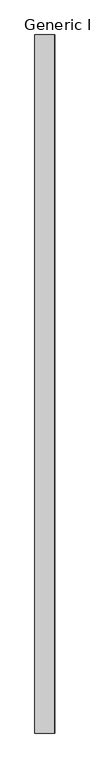
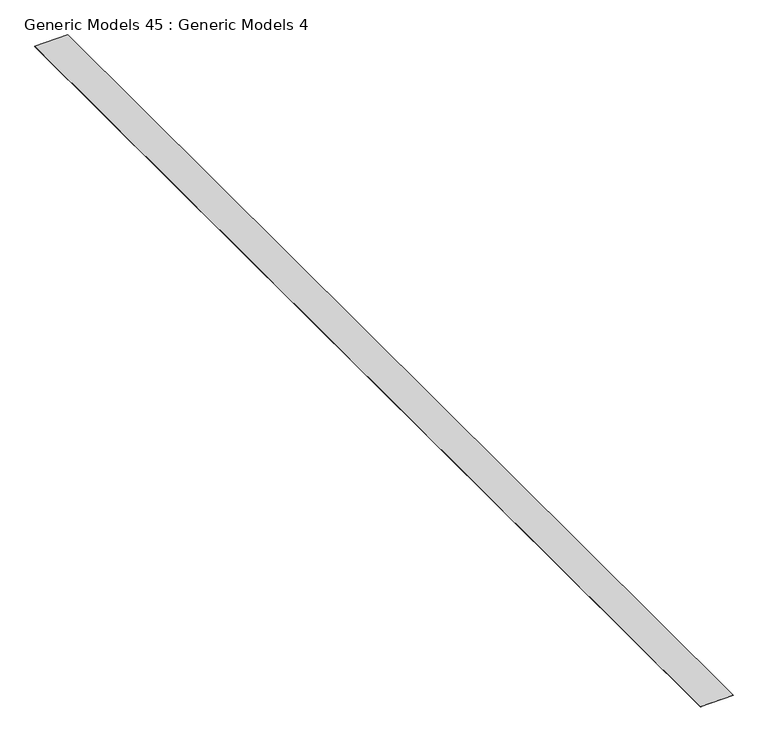
"""IFC4 building model written with IfcOpenShell, lengths in millimetres: proxy geometry, Generic Models 45 : Generic Models 4."""

from ifc_helpers import new_model, si_unit, frame, origin, place, context, project, spatial, polyline, outline, extrude, source, transform, mapped, element, save


def generic_models_45_generic_models_4_a326bbe1(model_context):
    return source(origin(), model_context, "Body", "SweptSolid", [
        extrude(outline(polyline([(0.0, -533.9447377), (0.0, 0.0), (18643.6, 0.0), (18643.6, -533.9447377), (0.0, -533.9447377)])), frame((7858.0260576, -6864.9230338, 126898.7093198), z_axis=(-0.02082881368186553, 0.0, 0.9997830567281115), x_axis=(0.0, 1.0, 0.0)), (0.0, 0.0, 1.0), 0.79375),
    ])


if __name__ == "__main__":
    model = new_model("IFC4")
    model_context = context("Model", 3, world=origin())
    ifc_project = project(units=[si_unit("LENGTHUNIT", "METRE", prefix="MILLI")], contexts=[model_context])
    site = spatial("IfcSite", under=ifc_project)
    building = spatial("IfcBuilding", under=site)
    placement = place(None, origin())
    generic_models_45_generic_models_4_shape = generic_models_45_generic_models_4_a326bbe1(model_context)
    element("IfcBuildingElementProxy", 1, Name="Generic Models 45 : Generic Models 4", ObjectType="Generic Models 45 : Generic Models 4", at=placement, inside=building, context=model_context, shape_type="MappedRepresentation", body=[
        mapped(generic_models_45_generic_models_4_shape, transform((0.0, 0.0, 0.0), x_axis=(1.0, 0.0, 0.0), y_axis=(0.0, 1.0, 0.0), z_axis=(0.0, 0.0, 1.0))),
    ])
    save(model, "model.ifc")

# Revit data of these elements
# Element 1 (IfcBuildingElementProxy, "Generic Models 45 : Generic Models 4")
#   Materials on its faces: "_HYDROSTOP LIQUID MEMBRANE - FOLLOW MANU. RECOMMENDED INSTALLATION DETAILS"
# Materials
#   "_HYDROSTOP LIQUID MEMBRANE - FOLLOW MANU. RECOMMENDED INSTALLATION DETAILS": class "Generic", colour RGB 156 184 169, transparency 0, Cost = 0
